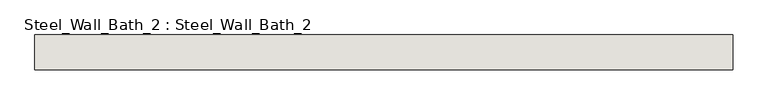
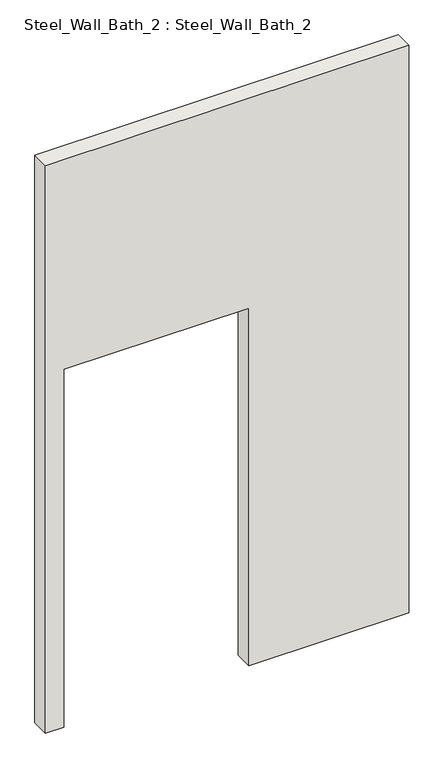
"""IFC4 building model written with IfcOpenShell, lengths in millimetres: wall geometry, Steel_Wall_Bath_2 : Steel_Wall_Bath_2."""

from ifc_helpers import new_model, si_unit, frame, origin, place, context, project, spatial, polyline, outline, extrude, source, transform, mapped, element, save


def steel_wall_bath_2_steel_wall_bath_2_118e7a6d(model_context):
    return source(origin(), model_context, "Body", "SweptSolid", [
        extrude(outline(polyline([(3550.0, 6075.0), (3550.0, 4075.0), (250.0, 4075.0), (250.0, 4175.0), (2330.0, 4175.0), (2330.0, 5195.0), (250.0, 5195.0), (250.0, 6075.0), (3550.0, 6075.0)])), frame((0.0, 14705.0, 0.0), z_axis=(0.0, 1.0, 0.0), x_axis=(0.0, 0.0, 1.0)), (0.0, 0.0, 1.0), 100.0),
    ])


if __name__ == "__main__":
    model = new_model("IFC4")
    model_context = context("Model", 3, world=origin())
    ifc_project = project(units=[si_unit("LENGTHUNIT", "METRE", prefix="MILLI")], contexts=[model_context])
    site = spatial("IfcSite", under=ifc_project)
    building = spatial("IfcBuilding", under=site)
    placement = place(None, origin())
    steel_wall_bath_2_steel_wall_bath_2_shape = steel_wall_bath_2_steel_wall_bath_2_118e7a6d(model_context)
    element("IfcWall", 1, ObjectType="Steel_Wall_Bath_2 : Steel_Wall_Bath_2", at=placement, inside=building, context=model_context, shape_type="MappedRepresentation", body=[
        mapped(steel_wall_bath_2_steel_wall_bath_2_shape, transform((0.0, 0.0, 0.0), x_axis=(1.0, 0.0, 0.0), y_axis=(0.0, 1.0, 0.0), z_axis=(0.0, 0.0, 1.0))),
    ])
    save(model, "model.ifc")

# Revit data of these elements
# Type "Steel_Wall_Bath_2 : Steel_Wall_Bath_2"
#   NameOverride = "Steel_Wall_Bath_2"
# Element 1 (IfcWall, "Steel_Wall_Bath_2 : Steel_Wall_Bath_2")
#   Materials on its faces: "IfcSurfaceStyle #33"
# Materials
#   "IfcSurfaceStyle #33": class "Unassigned", colour RGB 214 214 214, transparency 0
